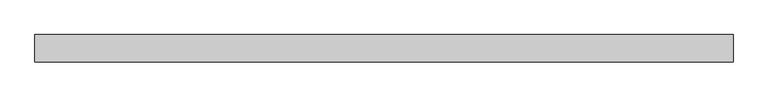
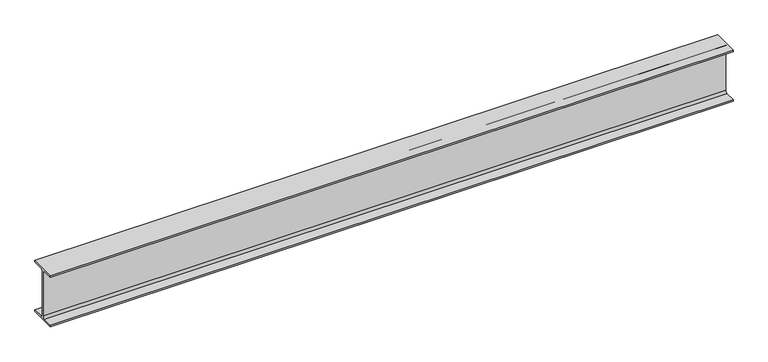
"""IFC4 building model written with IfcOpenShell, lengths in millimetres: beam geometry, 0912_Steel Framing_H-KSD3502 : H_SB_AR_S02_H-300x150x6.5x9_Stair."""

from ifc_helpers import new_model, si_unit, point, frame, frame_2d, origin, place, context, project, spatial, polyline, circle_curve, trimmed, segment, composite_curve, outline, extrude, source, transform, mapped, element, save


def beam_edbab3fa(model_context):
    return source(origin(), model_context, "Body", "SweptSolid", [
        extrude(outline(composite_curve([segment(polyline([(75.0, -141.0), (75.0, -150.0), (-75.0, -150.0), (-75.0, -141.0), (-16.25, -141.0)]), True, "CONTINUOUS"), segment(trimmed(circle_curve(frame_2d((-16.25, -128.0)), 13.0), [point((-16.25, -141.0))], [point((-3.25, -128.0))], True, "CARTESIAN"), True, "CONTINUOUS"), segment(polyline([(-3.25, -128.0), (-3.25, 128.0)]), True, "CONTINUOUS"), segment(trimmed(circle_curve(frame_2d((-16.25, 128.0)), 13.0), [point((-3.25, 128.0))], [point((-16.25, 141.0))], True, "CARTESIAN"), True, "CONTINUOUS"), segment(polyline([(-16.25, 141.0), (-75.0, 141.0), (-75.0, 150.0), (75.0, 150.0), (75.0, 141.0), (16.25, 141.0)]), True, "CONTINUOUS"), segment(trimmed(circle_curve(frame_2d((16.25, 128.0)), 13.0), [point((16.25, 141.0))], [point((3.25, 128.0))], True, "CARTESIAN"), True, "CONTINUOUS"), segment(polyline([(3.25, 128.0), (3.25, -128.0)]), True, "CONTINUOUS"), segment(trimmed(circle_curve(frame_2d((16.25, -128.0)), 13.0), [point((3.25, -128.0))], [point((16.25, -141.0))], True, "CARTESIAN"), True, "CONTINUOUS"), segment(polyline([(16.25, -141.0), (75.0, -141.0)]), True, "CONTINUOUS")], self_intersect=False)), frame((-1899.8, 0.0, 0.0), z_axis=(1.0, 0.0, 0.0), x_axis=(0.0, 1.0, 0.0)), (0.0, 0.0, 1.0), 3799.6),
    ])


if __name__ == "__main__":
    model = new_model("IFC4")
    model_context = context("Model", 3, world=origin())
    ifc_project = project(units=[si_unit("LENGTHUNIT", "METRE", prefix="MILLI")], contexts=[model_context])
    site = spatial("IfcSite", under=ifc_project)
    building = spatial("IfcBuilding", under=site)
    placement = place(None, origin())
    beam_shape = beam_edbab3fa(model_context)
    element("IfcBeam", 1, ObjectType="0912_Steel Framing_H-KSD3502 : H_SB_AR_S02_H-300x150x6.5x9_Stair", at=placement, inside=building, context=model_context, shape_type="MappedRepresentation", body=[
        mapped(beam_shape, transform((0.0, 0.0, 0.0), x_axis=(1.0, 0.0, 0.0), y_axis=(0.0, 1.0, 0.0), z_axis=(0.0, 0.0, 1.0))),
    ])
    save(model, "model.ifc")

# Revit data of these elements
# Type "0912_Steel Framing_H-KSD3502 : H_SB_AR_S02_H-300x150x6.5x9_Stair"
#   H_Q'ty Cal Type Tag = "SB-Q2"
#   H_WM Code_1 = "S01AA073-00001 |  | TON | Main Steel Structure Fabrication Work | Shelter/Building | Medium Steel - Standard |  |  |  |  |  |  | Material: (   ) | (90)KG/M>Weight≥(30)KG/M | S01AA073-00001 Main Steel Structure Fabrication Work Shelter/Building Medium Steel - Standard         | - Material: ( ASTM A36 )\n- (90)KG/M>Weight≥(30)KG/M"
#   H_WM Code_2 = "S03AA083-00001 |  | TON | Main Steel Structure Erection Work | Shelter/Building | Medium Steel |  |  |  |  |  |  | Material: (   ) | S03AA083-00001 Main Steel Structure Erection Work Shelter/Building Medium Steel         | - Material: ( ASTM A36 )"
#   H_WM Code_3 = "S01AA009-00001 |  | TON | Main Steel Structure Fabrication Work | Shelter/Building | Plates - Gusset, Stiffener, ETC | Material: (   ) | S01AA009-00001 Main Steel Structure Fabrication Work Shelter/Building Plates - Gusset, Stiffener, ETC         |"
#   H_WM Code_4 = "S41AA051-00001 |  | M2 | Steel Structure Paint Work | Shelter/Building | for Non-Fireproofed Steel Surface |  |  |  |  |  |  | Material: (   ) | S41AA051-00001 Steel Structure Paint Work Shelter/Building for Non-Fireproofed Steel Surface         |"
#   Width = 15.0 cm
#   Web Thickness = 0.65 cm
#   Web Fillet = 1.3 cm
#   Warping Constant = 107000.0 cm⁶
#   W = 0
#   Torsional Moment of Inertia = 9.9539 cm⁴
#   Section Area = 46.78 cm²
#   Plastic Modulus weak axis = 105.0 cm³
#   Plastic Modulus strong axis = 542.0 cm³
#   Perimeter = 1.17 m²/m
#   Nominal Weight = 36.70 kgf/m
#   Moment of Inertia weak axis = 508.00 cm⁴
#   Moment of Inertia strong axis = 7210.00 cm⁴
#   Height = 30.0 cm
#   Flange Thickness = 0.9 cm
#   Elastic Modulus weak axis = 67.7 cm³
#   Elastic Modulus strong axis = 481.0 cm³
#   Centroid Vertical = 15.0 cm
#   Centroid Horizontal = 7.5 cm
#   Ix = 72100000
#   Length [instance default] = 1524 mm
#   Zx = 542000
#   b = 150 mm
#   h = 300 mm
#   r = 13 mm
#   s = 6.5 mm
#   t = 9 mm
#   A = 0.004678 m²
#   Structural Material [instance default] = Steel, 45-345
#   Assembly Code = ""
# Element 1 (IfcBeam, "0912_Steel Framing_H-KSD3502 : H_SB_AR_S02_H-300x150x6.5x9_Stair")
#   Materials on its faces: "Steel, 45-345"
# Materials
#   "Steel, 45-345": class "Metal", colour RGB 189 187 185, transparency 0, Description = "Steel 345 MPa", Cost = 0
